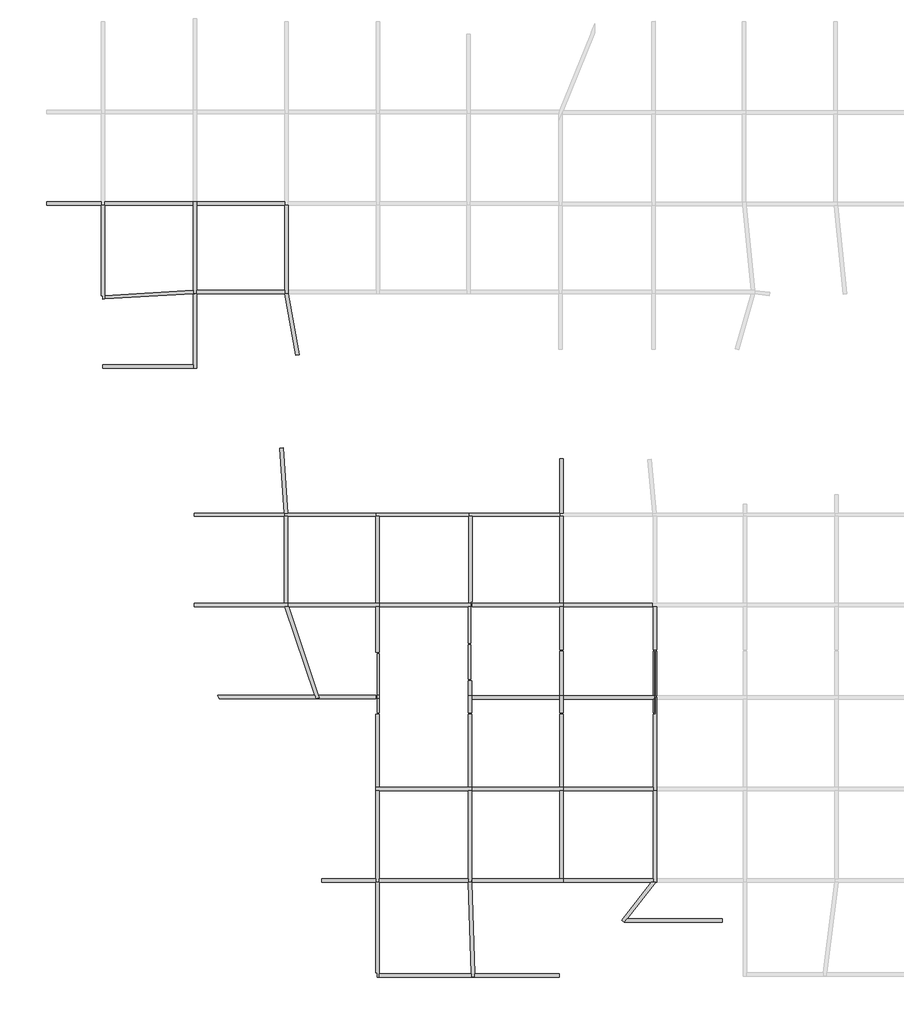
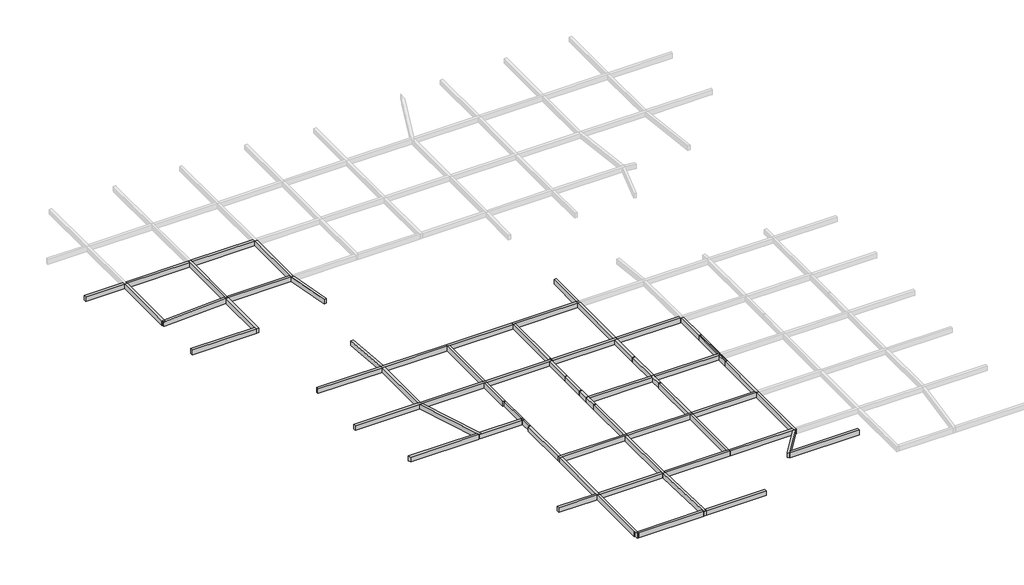
# One storey, part 1 of 8: 56 beams.
"""IFC4 building model written with IfcOpenShell, lengths in millimetres."""

import ifcopenshell
import ifcopenshell.guid

model = None  # the IFC model being written
_history = None  # IfcOwnerHistory: only IFC2X3 demands one
_inside = {}  # id of a spatial element -> (the spatial element, [elements in it])
_under = {}  # id of a project, library or spatial element -> (it, [spatial elements below it])
_declared = {}  # id of a project -> (the project, [libraries it declares])
_typed = {}  # id of a type object -> (the type object, [elements of that type])
_made_of = {}  # id of a material, layer set ... -> (it, [elements and type objects made of it])


def new_model(schema):
    """Start an empty IFC model of exactly this schema.

    Asked for "IFC4X3", IfcOpenShell would pick the latest addendum, in which some entities
    have other attributes; the version numbers below select the first issue.
    IFC2X3 requires an IfcOwnerHistory on every rooted entity: one is made here for all.
    """
    global model, _history
    if schema == "IFC4X3":
        model = ifcopenshell.file(schema_version=(4, 3, 0, 0))
    else:
        model = ifcopenshell.file(schema=schema)
    _inside.clear()
    _under.clear()
    _declared.clear()
    _typed.clear()
    _made_of.clear()
    _history = None
    if model.schema == "IFC2X3":
        org = make("IfcOrganization", Name="unknown")
        user = make(
            "IfcPersonAndOrganization",
            ThePerson=make("IfcPerson", FamilyName="unknown"),
            TheOrganization=org,
        )
        app = make(
            "IfcApplication",
            ApplicationDeveloper=org,
            Version="unknown",
            ApplicationFullName="unknown",
            ApplicationIdentifier="unknown",
        )
        _history = make(
            "IfcOwnerHistory",
            OwningUser=user,
            OwningApplication=app,
            ChangeAction="ADDED",
            CreationDate=0,
        )
    return model


def make(cls, **values):
    """One entity of the class cls with the attributes given. An attribute that is None is left unset."""
    return model.create_entity(
        cls, **{name: value for name, value in values.items() if value is not None}
    )


def rooted(cls, **values):
    """An entity with a GlobalId (a new one), such as an element, a storey or a relation."""
    return make(cls, GlobalId=ifcopenshell.guid.new(), OwnerHistory=_history, **values)


def si_unit(unit_type, name, prefix=None):
    """IfcSIUnit, for example si_unit("LENGTHUNIT", "METRE", prefix="MILLI")."""
    return make("IfcSIUnit", UnitType=unit_type, Prefix=prefix, Name=name)


def assignment(units):
    """IfcUnitAssignment: the units of a project."""
    return None if units is None else make("IfcUnitAssignment", Units=units)


def point(xyz):
    """IfcCartesianPoint."""
    return None if xyz is None else make("IfcCartesianPoint", Coordinates=xyz)


def direction(xyz):
    """IfcDirection."""
    return None if xyz is None else make("IfcDirection", DirectionRatios=xyz)


def frame(location, z_axis=None, x_axis=None):
    """IfcAxis2Placement3D, a coordinate frame: its origin and axes. An axis left out is left unset."""
    return make(
        "IfcAxis2Placement3D",
        Location=point(location),
        Axis=direction(z_axis),
        RefDirection=direction(x_axis),
    )


def origin():
    """The frame at (0, 0, 0) with its axes left unset."""
    return frame((0.0, 0.0, 0.0))


def place(relative_to, where):
    """IfcLocalPlacement: puts the frame where relative to a parent placement (None: the world)."""
    return make(
        "IfcLocalPlacement", PlacementRelTo=relative_to, RelativePlacement=where
    )


def context(
    kind, dimensions, precision=None, world=None, true_north=None, identifier=None
):
    """IfcGeometricRepresentationContext, for example the 3D "Model" context."""
    return make(
        "IfcGeometricRepresentationContext",
        ContextIdentifier=identifier,
        ContextType=kind,
        CoordinateSpaceDimension=dimensions,
        Precision=precision,
        WorldCoordinateSystem=world,
        TrueNorth=true_north,
    )


def project(units=None, contexts=None):
    """IfcProject with its units and contexts."""
    return rooted(
        "IfcProject",
        Name="project",
        RepresentationContexts=contexts,
        UnitsInContext=assignment(units),
    )


def spatial(cls, under=None, at=None, **own):
    """A site, building, storey or space (cls), placed at a placement, below another one or the project."""
    s = rooted(cls, ObjectPlacement=at, **own)
    if under is not None:
        _under.setdefault(under.id(), (under, []))[1].append(s)
    return s


def polyline(points):
    """IfcPolyline through the points."""
    return make("IfcPolyline", Points=[point(p) for p in points])


def outline(outer, holes=None, kind="AREA"):
    """IfcArbitraryClosedProfileDef: a profile drawn as a closed curve; with holes, ...WithVoids."""
    if holes is None:
        return make("IfcArbitraryClosedProfileDef", ProfileType=kind, OuterCurve=outer)
    return make(
        "IfcArbitraryProfileDefWithVoids",
        ProfileType=kind,
        OuterCurve=outer,
        InnerCurves=holes,
    )


def extrude(swept, where, along, depth):
    """IfcExtrudedAreaSolid: the profile swept, set in the frame where, extruded along a direction by depth."""
    return make(
        "IfcExtrudedAreaSolid",
        SweptArea=swept,
        Position=where,
        ExtrudedDirection=direction(along),
        Depth=depth,
    )


def faces_of(points, faces, orient=None, outer=None):
    """IfcFace entities. A face is a list of loops; a loop is a list of indices into points, from 0.

    orient and outer hold one flag for each loop. By default every Orientation is true, the
    first loop of a face is its IfcFaceOuterBound and the others are IfcFaceBound.
    """
    made = []
    for i, loops in enumerate(faces):
        bounds = []
        for j, loop in enumerate(loops):
            is_outer = j == 0 if outer is None else outer[i][j]
            bounds.append(
                make(
                    "IfcFaceOuterBound" if is_outer else "IfcFaceBound",
                    Bound=make("IfcPolyLoop", Polygon=[points[k] for k in loop]),
                    Orientation=True if orient is None else orient[i][j],
                )
            )
        made.append(make("IfcFace", Bounds=bounds))
    return made


def faceted_brep(points, faces, orient=None, outer=None, voids=None):
    """IfcFacetedBrep: a solid bounded by flat faces; with voids (closed shells), ...WithVoids."""
    shared = [point(p) for p in points]
    hull = make("IfcClosedShell", CfsFaces=faces_of(shared, faces, orient, outer))
    if voids is None:
        return make("IfcFacetedBrep", Outer=hull)
    return make(
        "IfcFacetedBrepWithVoids",
        Outer=hull,
        Voids=[
            make(cls, CfsFaces=faces_of(shared, fs, o, b)) for cls, fs, o, b in voids
        ],
    )


def shape(context_of_items, identifier, shape_type, items):
    """IfcShapeRepresentation: the items that make up one representation, for example the "Body"."""
    return make(
        "IfcShapeRepresentation",
        ContextOfItems=context_of_items,
        RepresentationIdentifier=identifier,
        RepresentationType=shape_type,
        Items=items,
    )


def made_of(thing, what):
    """Note that an element or type object is made of a material, layer set ...; save() writes the relation."""
    if what is not None:
        _made_of.setdefault(what.id(), (what, []))[1].append(thing)
    return thing


def element(
    cls,
    number,
    at=None,
    inside=None,
    cuts=None,
    type_object=None,
    material=None,
    context=None,
    identifier="Body",
    shape_type=None,
    held_by="IfcProductDefinitionShape",
    body=None,
    shapes=None,
    **own,
):
    """One element of the class cls, such as IfcWall. Its Tag is "e" and its number.

    at: its placement. inside: the storey or other place that contains it. cuts: it is an
    opening in that element (IfcRelVoidsElement). A single representation is given by context,
    identifier, shape_type and body (its items); several are given by shapes. held_by: the class
    of the entity that holds the representations. save() writes the other relations.
    """
    e = rooted(cls, Tag="e%d" % number, ObjectPlacement=at, **own)
    if body is not None:
        shapes = [shape(context, identifier, shape_type, body)]
    if shapes is not None:
        e.Representation = make(held_by, Representations=shapes)
    if inside is not None:
        _inside.setdefault(inside.id(), (inside, []))[1].append(e)
    if cuts is not None:
        rooted(
            "IfcRelVoidsElement", RelatingBuildingElement=cuts, RelatedOpeningElement=e
        )
    if type_object is not None:
        _typed.setdefault(type_object.id(), (type_object, []))[1].append(e)
    return made_of(e, material)


def aggregate(whole, parts):
    """IfcRelAggregates: a whole, such as a stair, and the parts it consists of."""
    return rooted("IfcRelAggregates", RelatingObject=whole, RelatedObjects=parts)


def save(model, path):
    """Write the relations noted so far, then the file.

    IfcRelAggregates (storeys below a building ...), IfcRelContainedInSpatialStructure (elements
    in a storey), IfcRelDefinesByType, IfcRelAssociatesMaterial and IfcRelDeclares: one each for
    every whole, place, type object, material and project.
    """
    for whole, parts in _under.values():
        aggregate(whole, parts)
    for where, things in _inside.values():
        rooted(
            "IfcRelContainedInSpatialStructure",
            RelatedElements=things,
            RelatingStructure=where,
        )
    for kind, things in _typed.values():
        rooted("IfcRelDefinesByType", RelatedObjects=things, RelatingType=kind)
    for what, things in _made_of.values():
        rooted("IfcRelAssociatesMaterial", RelatedObjects=things, RelatingMaterial=what)
    for by, libraries in _declared.values():
        rooted("IfcRelDeclares", RelatingContext=by, RelatedDefinitions=libraries)
    model.write(path)


model = new_model("IFC4")

# Units and contexts
model_context = context("Model", 3, world=origin())
ifc_project = project(units=[si_unit("LENGTHUNIT", "METRE", prefix="MILLI")], contexts=[model_context])

# Site, building, storey
site = spatial("IfcSite", under=ifc_project)
building = spatial("IfcBuilding", under=site)
storey = spatial("IfcBuildingStorey", under=building, Name="层高", Elevation=3300.0)

# Beams
placement = place(None, origin())
element("IfcBeam", 1, ObjectType="混凝土 - 矩形梁 : KL_beam", at=placement, inside=storey, context=model_context, shape_type="SweptSolid", body=[
    extrude(outline(polyline([(73233.8430954, 95377.0451941), (73233.8430954, 95677.0451941), (77970.8225114, 95677.0451941), (77970.8225114, 95377.0451941), (73233.8430954, 95377.0451941)])), frame((0.0, 0.0, 2700.0), z_axis=(0.0, 0.0, 1.0), x_axis=(1.0, 0.0, 0.0)), (0.0, 0.0, 1.0), 600.0),
])
element("IfcBeam", 2, ObjectType="混凝土 - 矩形梁 : KL_beam", at=placement, inside=storey, context=model_context, shape_type="Brep", body=[
    faceted_brep([(78270.8225114, 95377.0451941, 3300.0), (77970.8225114, 95377.0451941, 3300.0), (77970.8225114, 87547.0451941, 3300.0), (78083.8475536, 87547.0451941, 3300.0), (78083.8475536, 87427.0451941, 3300.0), (78083.8475536, 87285.4298587, 3300.0), (78270.8225114, 87285.4298587, 3300.0), (78270.8225114, 87585.9262923, 3300.0), (77970.8225114, 95377.0451941, 2700.0), (78270.8225114, 95377.0451941, 2700.0), (78270.8225114, 87585.9262923, 2700.0), (78270.8225114, 87285.4298587, 2700.0), (78083.8475536, 87285.4298587, 2700.0), (78083.8475536, 87547.0451941, 2700.0), (77970.8225114, 87547.0451941, 2700.0)], [[[0, 1, 2, 3, 4, 5, 6, 7]], [[8, 9, 10, 11, 12, 13, 14]], [[9, 0, 7, 6, 11, 10]], [[1, 0, 9, 8]], [[13, 3, 2, 14]], [[3, 13, 12, 5, 4]], [[11, 6, 5, 12]], [[1, 8, 14, 2]]]),
])
element("IfcBeam", 3, ObjectType="混凝土 - 矩形梁 : KL_beam", at=placement, inside=storey, context=model_context, shape_type="Brep", body=[
    faceted_brep([(86170.8225114, 95677.0451941, 3300.0), (85870.8225114, 95677.0451941, 3300.0), (85870.8225114, 95377.0451941, 3300.0), (85870.8225114, 88023.3256155, 3300.0), (85870.8225114, 87731.7102801, 3300.0), (86025.1353836, 87731.7102801, 3300.0), (86170.8225114, 87731.7102801, 3300.0), (86170.8225114, 88031.7102801, 3300.0), (86170.8225114, 95377.0451941, 3300.0), (86170.8225114, 95677.0451941, 2700.0), (86170.8225114, 87731.7102801, 2700.0), (86170.8225114, 88031.7102801, 2700.0), (86170.8225114, 95377.0451941, 2700.0), (85870.8225114, 95677.0451941, 2700.0), (86025.1353836, 87731.7102801, 2700.0), (85870.8225114, 87731.7102801, 2700.0), (85870.8225114, 88023.3256155, 2700.0), (85870.8225114, 95377.0451941, 2700.0)], [[[0, 1, 2, 3, 4, 5, 6, 7, 8]], [[9, 0, 8, 7, 6, 10, 11, 12]], [[13, 9, 12, 11, 10, 14, 15, 16, 17]], [[1, 13, 17, 16, 15, 4, 3, 2]], [[1, 0, 9, 13]], [[6, 5, 4, 15, 14, 10]]]),
])
element("IfcBeam", 4, ObjectType="混凝土 - 矩形梁 : KL_beam", at=placement, inside=storey, context=model_context, shape_type="Brep", body=[
    faceted_brep([(93770.8225114, 87731.7102801, 3300.0), (93794.9575667, 87731.7102801, 3300.0), (94070.8225114, 87731.7102801, 3300.0), (94070.8225114, 88031.7102801, 3300.0), (94070.8225114, 95377.0451941, 3300.0), (93770.8225114, 95377.0451941, 3300.0), (93770.8225114, 88031.7102801, 3300.0), (93770.8225114, 87731.7102801, 2700.0), (93770.8225114, 95377.0451941, 2700.0), (93770.8225114, 88031.7102801, 2700.0), (94070.8225114, 87731.7102801, 2700.0), (93794.9575667, 87731.7102801, 2700.0), (94070.8225114, 95377.0451941, 2700.0), (94070.8225114, 88031.7102801, 2700.0)], [[[0, 1, 2, 3, 4, 5, 6]], [[7, 0, 6, 5, 8, 9]], [[10, 11, 7, 9, 8, 12, 13]], [[2, 10, 13, 12, 4, 3]], [[5, 4, 12, 8]], [[2, 1, 0, 7, 11, 10]]]),
])
element("IfcBeam", 5, ObjectType="混凝土 - 矩形梁 : KL_beam", at=placement, inside=storey, context=model_context, shape_type="Brep", body=[
    faceted_brep([(109648.7128309, 68825.8567488, 3300.0), (109648.7128309, 68525.8567488, 3300.0), (109948.7128309, 68525.8567488, 3300.0), (117498.8477351, 68525.8567488, 3300.0), (117498.8477351, 68825.8567488, 3300.0), (109648.7128309, 68825.8567488, 2700.0), (117498.8477351, 68825.8567488, 2700.0), (109648.7128309, 68525.8567488, 2700.0), (117498.8477351, 68525.8567488, 2700.0), (109948.7128309, 68525.8567488, 2700.0)], [[[0, 1, 2, 3, 4]], [[5, 0, 4, 6]], [[7, 5, 6, 8, 9]], [[1, 7, 9, 8, 3, 2]], [[1, 0, 5, 7]], [[4, 3, 8, 6]]]),
])
element("IfcBeam", 6, ObjectType="混凝土 - 矩形梁 : KL_beam", at=placement, inside=storey, context=model_context, shape_type="Brep", body=[
    faceted_brep([(101648.7128309, 68825.8567488, 3300.0), (101648.7128309, 68525.8567488, 3300.0), (101948.7128309, 68525.8567488, 3300.0), (109648.7128309, 68525.8567488, 3300.0), (109648.7128309, 68825.8567488, 3300.0), (101648.7128309, 68825.8567488, 2700.0), (109648.7128309, 68825.8567488, 2700.0), (101648.7128309, 68525.8567488, 2700.0), (109648.7128309, 68525.8567488, 2700.0), (101948.7128309, 68525.8567488, 2700.0)], [[[0, 1, 2, 3, 4]], [[5, 0, 4, 6]], [[7, 5, 6, 8, 9]], [[1, 7, 9, 8, 3, 2]], [[4, 3, 8, 6]], [[1, 0, 5, 7]]]),
])
element("IfcBeam", 7, ObjectType="混凝土 - 矩形梁 : KL_beam", at=placement, inside=storey, context=model_context, shape_type="Brep", body=[
    faceted_brep([(93748.7128309, 68825.8567488, 3300.0), (93748.7128309, 68525.8567488, 3300.0), (94048.7128309, 68525.8567488, 3300.0), (101648.7128309, 68525.8567488, 3300.0), (101648.7128309, 68825.8567488, 3300.0), (94038.5900938, 68825.8567488, 3300.0), (93748.7128309, 68825.8567488, 2700.0), (101648.7128309, 68825.8567488, 2700.0), (94038.5900938, 68825.8567488, 2700.0), (93748.7128309, 68525.8567488, 2700.0), (101648.7128309, 68525.8567488, 2700.0), (94048.7128309, 68525.8567488, 2700.0)], [[[0, 1, 2, 3, 4, 5]], [[6, 0, 5, 4, 7, 8]], [[9, 6, 8, 7, 10, 11]], [[1, 9, 11, 10, 3, 2]], [[4, 3, 10, 7]], [[1, 0, 6, 9]]]),
])
element("IfcBeam", 8, ObjectType="混凝土 - 矩形梁 : KL_beam", at=placement, inside=storey, context=model_context, shape_type="Brep", body=[
    faceted_brep([(85958.8477345, 68825.8567488, 3300.0), (85958.8477345, 68525.8567488, 3300.0), (93748.7128309, 68525.8567488, 3300.0), (93748.7128309, 68825.8567488, 3300.0), (93737.8575244, 68825.8567488, 3300.0), (85958.8477345, 68825.8567488, 2700.0), (93748.7128309, 68825.8567488, 2700.0), (93737.8575244, 68825.8567488, 2700.0), (85958.8477345, 68525.8567488, 2700.0), (93748.7128309, 68525.8567488, 2700.0)], [[[0, 1, 2, 3, 4]], [[5, 0, 4, 3, 6, 7]], [[8, 5, 7, 6, 9]], [[1, 8, 9, 2]], [[1, 0, 5, 8]], [[3, 2, 9, 6]]]),
])
element("IfcBeam", 9, ObjectType="混凝土 - 矩形梁 : KL_beam", at=placement, inside=storey, context=model_context, shape_type="Brep", body=[
    faceted_brep([(94048.7128309, 60727.1438632, 3300.0), (94048.7128309, 61027.1438632, 3300.0), (93748.7128309, 61027.1438632, 3300.0), (85958.8477345, 61027.1438632, 3300.0), (85958.8477345, 60727.1438632, 3300.0), (93791.0953712, 60727.1438632, 3300.0), (94048.7128309, 60727.1438632, 2700.0), (85958.8477345, 60727.1438632, 2700.0), (93791.0953712, 60727.1438632, 2700.0), (94048.7128309, 61027.1438632, 2700.0), (85958.8477345, 61027.1438632, 2700.0), (93748.7128309, 61027.1438632, 2700.0)], [[[0, 1, 2, 3, 4, 5]], [[6, 0, 5, 4, 7, 8]], [[9, 6, 8, 7, 10, 11]], [[1, 9, 11, 10, 3, 2]], [[4, 3, 10, 7]], [[1, 0, 6, 9]]]),
])
element("IfcBeam", 10, ObjectType="混凝土 - 矩形梁 : KL_beam", at=placement, inside=storey, context=model_context, shape_type="Brep", body=[
    faceted_brep([(101948.7128309, 60727.1438632, 3300.0), (101948.7128309, 61027.1438632, 3300.0), (101648.7128309, 61027.1438632, 3300.0), (94048.7128309, 61027.1438632, 3300.0), (94048.7128309, 60727.1438632, 3300.0), (94107.7867122, 60727.1438632, 3300.0), (101648.7128309, 60727.1438632, 3300.0), (101948.7128309, 60727.1438632, 2700.0), (94048.7128309, 60727.1438632, 2700.0), (94107.7867122, 60727.1438632, 2700.0), (101648.7128309, 60727.1438632, 2700.0), (101948.7128309, 61027.1438632, 2700.0), (94048.7128309, 61027.1438632, 2700.0), (101648.7128309, 61027.1438632, 2700.0)], [[[0, 1, 2, 3, 4, 5, 6]], [[7, 0, 6, 5, 4, 8, 9, 10]], [[11, 7, 10, 9, 8, 12, 13]], [[1, 11, 13, 12, 3, 2]], [[1, 0, 7, 11]], [[4, 3, 12, 8]]]),
])
element("IfcBeam", 11, ObjectType="混凝土 - 矩形梁 : KL_beam", at=placement, inside=storey, context=model_context, shape_type="Brep", body=[
    faceted_brep([(101948.7128309, 61027.1438632, 3300.0), (101948.7128309, 60727.1438632, 3300.0), (109598.8477351, 60727.1438632, 3300.0), (109838.7128377, 60727.1438632, 3300.0), (109838.7128377, 61027.1438632, 3300.0), (109648.7128309, 61027.1438632, 3300.0), (101948.7128309, 60727.1438632, 2700.0), (109598.8477351, 60727.1438632, 2700.0), (109838.7128377, 60727.1438632, 2700.0), (101948.7128309, 61027.1438632, 2700.0), (109648.7128309, 61027.1438632, 2700.0), (109838.7128377, 61027.1438632, 2700.0)], [[[0, 1, 2, 3, 4, 5]], [[1, 6, 7, 8, 3, 2]], [[6, 9, 10, 11, 8, 7]], [[9, 0, 5, 4, 11, 10]], [[1, 0, 9, 6]], [[4, 3, 8, 11]]]),
])
element("IfcBeam", 12, ObjectType="混凝土 - 矩形梁 : KL_beam", at=placement, inside=storey, context=model_context, shape_type="Brep", body=[
    faceted_brep([(117798.8477351, 60727.1438632, 3300.0), (117798.8477351, 61027.1438632, 3300.0), (117498.8477351, 61027.1438632, 3300.0), (109958.7128377, 61027.1438632, 3300.0), (109958.7128377, 60727.1438632, 3300.0), (117498.8477351, 60727.1438632, 3300.0), (117798.8477351, 60727.1438632, 2700.0), (109958.7128377, 60727.1438632, 2700.0), (117498.8477351, 60727.1438632, 2700.0), (117798.8477351, 61027.1438632, 2700.0), (109958.7128377, 61027.1438632, 2700.0), (117498.8477351, 61027.1438632, 2700.0)], [[[0, 1, 2, 3, 4, 5]], [[6, 0, 5, 4, 7, 8]], [[9, 6, 8, 7, 10, 11]], [[1, 9, 11, 10, 3, 2]], [[1, 0, 6, 9]], [[4, 3, 10, 7]]]),
])
element("IfcBeam", 13, ObjectType="混凝土 - 矩形梁 : KL_beam", at=placement, inside=storey, context=model_context, shape_type="SweptSolid", body=[
    extrude(outline(polyline([(125476.4248507, 61027.1438632), (125476.4248507, 60727.1438632), (117798.8477351, 60727.1438632), (117798.8477351, 61027.1438632), (125476.4248507, 61027.1438632)])), frame((0.0, 0.0, 2700.0), z_axis=(0.0, 0.0, 1.0), x_axis=(1.0, 0.0, 0.0)), (0.0, 0.0, 1.0), 600.0),
])
element("IfcBeam", 14, ObjectType="混凝土 - 矩形梁 : KL_beam", at=placement, inside=storey, context=model_context, shape_type="SweptSolid", body=[
    extrude(outline(polyline([(109648.7128309, 68525.8567488), (109948.7128309, 68525.8567488), (109948.7128309, 61154.2483952), (109838.7128377, 61154.2483952), (109838.7128377, 61027.1438632), (109648.7128309, 61027.1438632), (109648.7128309, 68525.8567488)])), frame((0.0, 0.0, 2700.0), z_axis=(0.0, 0.0, 1.0), x_axis=(1.0, 0.0, 0.0)), (0.0, 0.0, 1.0), 600.0),
])
element("IfcBeam", 15, ObjectType="混凝土 - 矩形梁 : KL_beam", at=placement, inside=storey, context=model_context, shape_type="SweptSolid", body=[
    extrude(outline(polyline([(101648.7128309, 68525.8567488), (101948.7128309, 68525.8567488), (101948.7128309, 61027.1438632), (101648.7128309, 61027.1438632), (101648.7128309, 68525.8567488)])), frame((0.0, 0.0, 2700.0), z_axis=(0.0, 0.0, 1.0), x_axis=(1.0, 0.0, 0.0)), (0.0, 0.0, 1.0), 600.0),
])
element("IfcBeam", 16, ObjectType="混凝土 - 矩形梁 : KL_beam", at=placement, inside=storey, context=model_context, shape_type="SweptSolid", body=[
    extrude(outline(polyline([(93748.7128309, 68525.8567488), (94048.7128309, 68525.8567488), (94048.7128309, 61027.1438632), (93748.7128309, 61027.1438632), (93748.7128309, 68525.8567488)])), frame((0.0, 0.0, 2700.0), z_axis=(0.0, 0.0, 1.0), x_axis=(1.0, 0.0, 0.0)), (0.0, 0.0, 1.0), 600.0),
])
element("IfcBeam", 17, ObjectType="混凝土 - 矩形梁 : KL_beam", at=placement, inside=storey, context=model_context, shape_type="Brep", body=[
    faceted_brep([(93345.7815071, 74432.8050195, 3300.0), (93645.0507222, 74453.7319616, 3300.0), (93645.0507222, 74453.7319616, 2700.0), (93345.7815071, 74432.8050195, 2700.0), (93737.8575244, 68825.8567488, 3300.0), (93748.7128309, 68825.8567488, 3300.0), (94038.5900938, 68825.8567488, 3300.0), (94038.5900938, 68825.8567488, 2700.0), (93748.7128309, 68825.8567488, 2700.0), (93737.8575244, 68825.8567488, 2700.0)], [[[0, 1, 2, 3]], [[1, 0, 4, 5, 6]], [[2, 1, 6, 7]], [[3, 2, 7, 8, 9]], [[0, 3, 9, 4]], [[4, 9, 8, 7, 6, 5]]]),
])
element("IfcBeam", 18, ObjectType="混凝土 - 矩形梁 : KL_beam", at=placement, inside=storey, context=model_context, shape_type="Brep", body=[
    faceted_brep([(94107.7867122, 60727.1438632, 3300.0), (94048.7128309, 60727.1438632, 3300.0), (93791.0953712, 60727.1438632, 3300.0), (96364.7738589, 53116.9449825, 3300.0), (96466.2302805, 52816.9449825, 3300.0), (96750.4186632, 52913.0541037, 3300.0), (96681.4652, 53116.9449825, 3300.0), (93791.0953712, 60727.1438632, 2700.0), (96364.7738589, 53116.9449825, 2700.0), (96466.2302805, 52816.9449825, 2700.0), (94048.7128309, 60727.1438632, 2700.0), (94107.7867122, 60727.1438632, 2700.0), (96681.4652, 53116.9449825, 2700.0), (96750.4186632, 52913.0541037, 2700.0)], [[[0, 1, 2, 3, 4, 5, 6]], [[4, 3, 2, 7, 8, 9]], [[9, 8, 7, 10, 11, 12, 13]], [[5, 13, 12, 11, 0, 6]], [[0, 11, 10, 7, 2, 1]], [[5, 4, 9, 13]]]),
])
element("IfcBeam", 19, ObjectType="混凝土 - 矩形梁 : KL_beam", at=placement, inside=storey, context=model_context, shape_type="Brep", body=[
    faceted_brep([(88137.9209142, 52816.9449825, 3300.0), (96423.8477403, 52816.9449825, 3300.0), (96466.2302805, 52816.9449825, 3300.0), (96364.7738589, 53116.9449825, 3300.0), (88016.7130465, 53116.9449825, 3300.0), (88016.7130465, 53116.9449825, 2700.0), (96364.7738589, 53116.9449825, 2700.0), (96466.2302805, 52816.9449825, 2700.0), (96423.8477403, 52816.9449825, 2700.0), (88137.9209142, 52816.9449825, 2700.0)], [[[0, 1, 2, 3, 4]], [[5, 4, 3, 6]], [[7, 8, 9, 5, 6]], [[2, 1, 0, 9, 8, 7]], [[0, 4, 5, 9]], [[3, 2, 7, 6]]]),
])
element("IfcBeam", 20, ObjectType="混凝土 - 矩形梁 : KL_beam", at=placement, inside=storey, context=model_context, shape_type="Brep", body=[
    faceted_brep([(101948.7128309, 52816.9449825, 3300.0), (101948.7128309, 53116.9449825, 3300.0), (101758.8477337, 53116.9449825, 3300.0), (101758.8477337, 52816.9449825, 3300.0), (101948.7128309, 52816.9449825, 2700.0), (101758.8477337, 52816.9449825, 2700.0), (101948.7128309, 53116.9449825, 2700.0), (101758.8477337, 53116.9449825, 2700.0)], [[[0, 1, 2, 3]], [[4, 0, 3, 5]], [[6, 4, 5, 7]], [[1, 6, 7, 2]], [[1, 0, 4, 6]], [[3, 2, 7, 5]]]),
    faceted_brep([(96750.4186632, 52913.0541037, 2700.0), (96750.4186632, 52913.0541037, 3300.0), (96681.4652, 53116.9449825, 3300.0), (96681.4652, 53116.9449825, 2700.0), (96466.2302805, 52816.9449825, 2700.0), (96466.2302805, 52816.9449825, 3300.0), (101638.8477337, 53116.9449825, 3300.0), (101638.8477337, 52816.9449825, 3300.0), (101638.8477337, 52816.9449825, 2700.0), (101638.8477337, 53116.9449825, 2700.0), (96723.8477403, 52816.9449825, 3300.0), (96723.8477403, 52816.9449825, 2700.0)], [[[0, 1, 2, 3]], [[1, 0, 4, 5]], [[6, 7, 8, 9]], [[2, 1, 5, 10, 7, 6]], [[5, 4, 11, 8, 7, 10]], [[0, 3, 9, 8, 11, 4]], [[3, 2, 6, 9]]]),
])
element("IfcBeam", 21, ObjectType="混凝土 - 矩形梁 : KL_beam", at=placement, inside=storey, context=model_context, shape_type="Brep", body=[
    faceted_brep([(109898.8477351, 44882.6668088, 3300.0), (109898.8477351, 45182.6668088, 3300.0), (109598.8477351, 45182.6668088, 3300.0), (101948.7128309, 45182.6668088, 3300.0), (101648.7128309, 45182.6668088, 3300.0), (101648.7128309, 44882.6668088, 3300.0), (101948.7128309, 44882.6668088, 3300.0), (109598.8477351, 44882.6668088, 3300.0), (109898.8477351, 44882.6668088, 2700.0), (101648.7128309, 44882.6668088, 2700.0), (101948.7128309, 44882.6668088, 2700.0), (109598.8477351, 44882.6668088, 2700.0), (109898.8477351, 45182.6668088, 2700.0), (101648.7128309, 45182.6668088, 2700.0), (101948.7128309, 45182.6668088, 2700.0), (109598.8477351, 45182.6668088, 2700.0)], [[[0, 1, 2, 3, 4, 5, 6, 7]], [[8, 0, 7, 6, 5, 9, 10, 11]], [[12, 8, 11, 10, 9, 13, 14, 15]], [[1, 12, 15, 14, 13, 4, 3, 2]], [[1, 0, 8, 12]], [[5, 4, 13, 9]]]),
])
element("IfcBeam", 22, ObjectType="混凝土 - 矩形梁 : KL_beam", at=placement, inside=storey, context=model_context, shape_type="Brep", body=[
    faceted_brep([(109898.8477351, 53082.6668088, 3300.0), (109598.8477351, 53082.6668088, 3300.0), (109598.8477351, 52816.9449825, 3300.0), (109598.8477351, 51576.8472247, 3300.0), (109898.8477351, 51576.8472247, 3300.0), (109898.8477351, 52782.6668088, 3300.0), (109898.8477351, 53082.6668088, 2700.0), (109898.8477351, 51576.8472247, 2700.0), (109898.8477351, 52782.6668088, 2700.0), (109598.8477351, 53082.6668088, 2700.0), (109598.8477351, 51576.8472247, 2700.0), (109598.8477351, 52816.9449825, 2700.0)], [[[0, 1, 2, 3, 4, 5]], [[6, 0, 5, 4, 7, 8]], [[9, 6, 8, 7, 10, 11]], [[1, 9, 11, 10, 3, 2]], [[1, 0, 6, 9]], [[4, 3, 10, 7]]]),
    faceted_brep([(109898.8477351, 45182.6668088, 3300.0), (109598.8477351, 45182.6668088, 3300.0), (109598.8477351, 45182.6668088, 2700.0), (109898.8477351, 45182.6668088, 2700.0), (109598.8477351, 51456.8472247, 3300.0), (109898.8477351, 51456.8472247, 3300.0), (109898.8477351, 51456.8472247, 2700.0), (109598.8477351, 51456.8472247, 2700.0)], [[[0, 1, 2, 3]], [[4, 5, 6, 7]], [[1, 0, 5, 4]], [[0, 3, 6, 5]], [[3, 2, 7, 6]], [[2, 1, 4, 7]]]),
])
element("IfcBeam", 23, ObjectType="混凝土 - 矩形梁 : KL_beam", at=placement, inside=storey, context=model_context, shape_type="Brep", body=[
    faceted_brep([(109598.8477351, 60727.1438632, 3300.0), (109598.8477351, 57577.1438632, 3300.0), (109838.7128377, 57577.1438632, 3300.0), (109838.7128377, 60727.1438632, 3300.0), (109598.8477351, 57577.1438632, 2700.0), (109598.8477351, 60727.1438632, 2700.0), (109838.7128377, 60727.1438632, 2700.0), (109838.7128377, 57577.1438632, 2700.0)], [[[0, 1, 2, 3]], [[4, 5, 6, 7]], [[0, 5, 4, 1]], [[5, 0, 3, 6]], [[2, 1, 4, 7]], [[3, 2, 7, 6]]]),
    faceted_brep([(109898.8477351, 53082.6668088, 3300.0), (109898.8477351, 53082.6668088, 2700.0), (109898.8477351, 54367.0649839, 2700.0), (109898.8477351, 54367.0649839, 3300.0), (109598.8477351, 53082.6668088, 3300.0), (109598.8477351, 53082.6668088, 2700.0), (109598.8477351, 54367.0649839, 2700.0), (109598.8477351, 54367.0649839, 3300.0), (109598.8477351, 53116.9449825, 3300.0), (109598.8477351, 53116.9449825, 2700.0)], [[[0, 1, 2, 3]], [[0, 4, 5, 1]], [[3, 2, 6, 7]], [[5, 4, 8, 7, 6, 9]], [[4, 0, 3, 7, 8]], [[1, 5, 9, 6, 2]]]),
    faceted_brep([(109598.8477351, 57457.1438632, 3300.0), (109838.7128377, 57457.1438632, 3300.0), (109838.7128377, 57457.1438632, 2700.0), (109598.8477351, 57457.1438632, 2700.0), (109598.8477351, 54487.0649839, 2700.0), (109598.8477351, 54487.0649839, 3300.0), (109838.7128377, 54487.0649839, 3300.0), (109838.7128377, 54487.0649839, 2700.0)], [[[0, 1, 2, 3]], [[0, 3, 4, 5]], [[1, 0, 5, 6]], [[3, 2, 7, 4]], [[1, 6, 7, 2]], [[5, 4, 7, 6]]]),
])
element("IfcBeam", 24, ObjectType="混凝土 - 矩形梁 : KL_beam", at=placement, inside=storey, context=model_context, shape_type="SweptSolid", body=[
    extrude(outline(polyline([(101948.7128309, 56681.8460485), (101948.7128309, 53116.9449825), (101758.8477337, 53116.9449825), (101758.8477337, 56681.8460485), (101948.7128309, 56681.8460485)])), frame((0.0, 0.0, 2700.0), z_axis=(0.0, 0.0, 1.0), x_axis=(1.0, 0.0, 0.0)), (0.0, 0.0, 1.0), 600.0),
    extrude(outline(polyline([(101648.7128309, 60727.1438632), (101948.7128309, 60727.1438632), (101948.7128309, 56801.8460485), (101648.7128309, 56801.8460485), (101648.7128309, 60727.1438632)])), frame((0.0, 0.0, 2700.0), z_axis=(0.0, 0.0, 1.0), x_axis=(1.0, 0.0, 0.0)), (0.0, 0.0, 1.0), 600.0),
])
element("IfcBeam", 25, ObjectType="混凝土 - 矩形梁 : KL_beam", at=placement, inside=storey, context=model_context, shape_type="SweptSolid", body=[
    extrude(outline(polyline([(101948.7128309, 45182.6668088), (101648.7128309, 45182.6668088), (101648.7128309, 51456.8472247), (101948.7128309, 51456.8472247), (101948.7128309, 45182.6668088)])), frame((0.0, 0.0, 2700.0), z_axis=(0.0, 0.0, 1.0), x_axis=(1.0, 0.0, 0.0)), (0.0, 0.0, 1.0), 600.0),
    extrude(outline(polyline([(101948.7128309, 52816.9449825), (101948.7128309, 51576.8472247), (101758.8477337, 51576.8472247), (101758.8477337, 52816.9449825), (101948.7128309, 52816.9449825)])), frame((0.0, 0.0, 2700.0), z_axis=(0.0, 0.0, 1.0), x_axis=(1.0, 0.0, 0.0)), (0.0, 0.0, 1.0), 600.0),
])
element("IfcBeam", 26, ObjectType="混凝土 - 矩形梁 : KL_beam", at=placement, inside=storey, context=model_context, shape_type="Brep", body=[
    faceted_brep([(101648.7128309, 36982.6668088, 3300.0), (101948.7128309, 36982.6668088, 3300.0), (101948.7128309, 37282.6668088, 3300.0), (101948.7128309, 44882.6668088, 3300.0), (101648.7128309, 44882.6668088, 3300.0), (101648.7128309, 37282.6668088, 3300.0), (101648.7128309, 36982.6668088, 2700.0), (101648.7128309, 44882.6668088, 2700.0), (101648.7128309, 37282.6668088, 2700.0), (101948.7128309, 36982.6668088, 2700.0), (101948.7128309, 44882.6668088, 2700.0), (101948.7128309, 37282.6668088, 2700.0)], [[[0, 1, 2, 3, 4, 5]], [[6, 0, 5, 4, 7, 8]], [[9, 6, 8, 7, 10, 11]], [[1, 9, 11, 10, 3, 2]], [[4, 3, 10, 7]], [[1, 0, 6, 9]]]),
])
element("IfcBeam", 27, ObjectType="混凝土 - 矩形梁 : KL_beam", at=placement, inside=storey, context=model_context, shape_type="Brep", body=[
    faceted_brep([(101648.7128309, 29151.649632, 3300.0), (101758.8477432, 29151.649632, 3300.0), (101758.8477432, 29031.649632, 3300.0), (101758.8477432, 28766.8473862, 3300.0), (101948.7128309, 28766.8473862, 3300.0), (101948.7128309, 29066.8473862, 3300.0), (101948.7128309, 36982.6668088, 3300.0), (101648.7128309, 36982.6668088, 3300.0), (101758.8477432, 28766.8473862, 2700.0), (101758.8477432, 29151.649632, 2700.0), (101648.7128309, 29151.649632, 2700.0), (101648.7128309, 36982.6668088, 2700.0), (101948.7128309, 36982.6668088, 2700.0), (101948.7128309, 29066.8473862, 2700.0), (101948.7128309, 28766.8473862, 2700.0)], [[[0, 1, 2, 3, 4, 5, 6, 7]], [[8, 9, 10, 11, 12, 13, 14]], [[12, 6, 5, 4, 14, 13]], [[9, 1, 0, 10]], [[1, 9, 8, 3, 2]], [[10, 0, 7, 11]], [[7, 6, 12, 11]], [[14, 4, 3, 8]]]),
])
element("IfcBeam", 28, ObjectType="混凝土 - 矩形梁 : KL_beam", at=placement, inside=storey, context=model_context, shape_type="SweptSolid", body=[
    extrude(outline(polyline([(96978.261361, 36982.6668088), (96978.261361, 37282.6668088), (101648.7128309, 37282.6668088), (101648.7128309, 36982.6668088), (96978.261361, 36982.6668088)])), frame((0.0, 0.0, 2700.0), z_axis=(0.0, 0.0, 1.0), x_axis=(1.0, 0.0, 0.0)), (0.0, 0.0, 1.0), 600.0),
])
element("IfcBeam", 29, ObjectType="混凝土 - 矩形梁 : KL_beam", at=placement, inside=storey, context=model_context, shape_type="Brep", body=[
    faceted_brep([(109598.8477351, 36982.6668088, 3300.0), (109603.6768872, 36982.6668088, 3300.0), (109898.8477351, 36982.6668088, 3300.0), (109898.8477351, 37135.1208886, 3300.0), (109898.8477351, 37282.6668088, 3300.0), (109898.8477351, 44882.6668088, 3300.0), (109598.8477351, 44882.6668088, 3300.0), (109598.8477351, 37282.6668088, 3300.0), (109598.8477351, 36982.6668088, 2700.0), (109598.8477351, 44882.6668088, 2700.0), (109598.8477351, 37282.6668088, 2700.0), (109898.8477351, 36982.6668088, 2700.0), (109603.6768872, 36982.6668088, 2700.0), (109898.8477351, 44882.6668088, 2700.0), (109898.8477351, 37282.6668088, 2700.0), (109898.8477351, 37135.1208886, 2700.0)], [[[0, 1, 2, 3, 4, 5, 6, 7]], [[8, 0, 7, 6, 9, 10]], [[11, 12, 8, 10, 9, 13, 14, 15]], [[2, 11, 15, 14, 13, 5, 4, 3]], [[6, 5, 13, 9]], [[2, 1, 0, 8, 12, 11]]]),
])
element("IfcBeam", 30, ObjectType="混凝土 - 矩形梁 : KL_beam", at=placement, inside=storey, context=model_context, shape_type="SweptSolid", body=[
    extrude(outline(polyline([(101948.7128309, 36982.6668088), (101948.7128309, 37282.6668088), (109598.8477351, 37282.6668088), (109598.8477351, 36982.6668088), (101948.7128309, 36982.6668088)])), frame((0.0, 0.0, 2700.0), z_axis=(0.0, 0.0, 1.0), x_axis=(1.0, 0.0, 0.0)), (0.0, 0.0, 1.0), 600.0),
])
element("IfcBeam", 31, ObjectType="混凝土 - 矩形梁 : KL_beam", at=placement, inside=storey, context=model_context, shape_type="Brep", body=[
    faceted_brep([(110172.4186602, 28776.6610787, 3300.0), (110162.9209132, 29066.8473862, 3300.0), (109903.8375304, 36982.6668088, 3300.0), (109898.8477351, 37135.1208886, 3300.0), (109898.8477351, 36982.6668088, 3300.0), (109603.6768872, 36982.6668088, 3300.0), (109862.76027, 29066.8473862, 3300.0), (109872.5792174, 28766.8473862, 3300.0), (109603.6768872, 36982.6668088, 2700.0), (109862.76027, 29066.8473862, 2700.0), (109872.5792174, 28766.8473862, 2700.0), (109898.8477351, 36982.6668088, 2700.0), (109898.8477351, 37135.1208886, 2700.0), (109903.8375304, 36982.6668088, 2700.0), (110162.9209132, 29066.8473862, 2700.0), (110172.4186602, 28776.6610787, 2700.0)], [[[0, 1, 2, 3, 4, 5, 6, 7]], [[7, 6, 5, 8, 9, 10]], [[10, 9, 8, 11, 12, 13, 14, 15]], [[3, 2, 1, 0, 15, 14, 13, 12]], [[11, 4, 3, 12]], [[4, 11, 8, 5]], [[0, 7, 10, 15]]]),
])
element("IfcBeam", 32, ObjectType="混凝土 - 矩形梁 : KL_beam", at=placement, inside=storey, context=model_context, shape_type="Brep", body=[
    faceted_brep([(101948.7128309, 29066.8473862, 3300.0), (101948.7128309, 28766.8473862, 3300.0), (109872.5792174, 28766.8473862, 3300.0), (109862.76027, 29066.8473862, 3300.0), (101948.7128309, 29066.8473862, 2700.0), (109862.76027, 29066.8473862, 2700.0), (101948.7128309, 28766.8473862, 2700.0), (109872.5792174, 28766.8473862, 2700.0), (110172.7398606, 28766.8473862, 2700.0), (110172.7398606, 28766.8473862, 3300.0), (110172.4186602, 28776.6610787, 2700.0), (110172.4186602, 28776.6610787, 3300.0)], [[[0, 1, 2, 3]], [[4, 0, 3, 5]], [[6, 4, 5, 7]], [[8, 9, 2, 1, 6, 7]], [[9, 8, 10, 11]], [[1, 0, 4, 6]], [[2, 7, 5, 3]], [[7, 2, 11, 10]], [[9, 11, 2]], [[10, 8, 7]]]),
])
element("IfcBeam", 33, ObjectType="混凝土 - 矩形梁 : KL_beam", at=placement, inside=storey, context=model_context, shape_type="Brep", body=[
    faceted_brep([(117798.8477351, 36982.6668088, 3300.0), (117798.8477351, 37282.6668088, 3300.0), (117498.8477351, 37282.6668088, 3300.0), (109898.8477351, 37282.6668088, 3300.0), (109898.8477351, 37135.1208886, 3300.0), (109903.8375304, 36982.6668088, 3300.0), (117798.8477351, 36982.6668088, 2700.0), (109903.8375304, 36982.6668088, 2700.0), (117798.8477351, 37282.6668088, 2700.0), (109898.8477351, 37135.1208886, 2700.0), (109898.8477351, 37282.6668088, 2700.0), (117498.8477351, 37282.6668088, 2700.0)], [[[0, 1, 2, 3, 4, 5]], [[6, 0, 5, 7]], [[8, 6, 7, 9, 10, 11]], [[10, 3, 2, 1, 8, 11]], [[3, 10, 9, 4]], [[5, 4, 9, 7]], [[1, 0, 6, 8]]]),
])
element("IfcBeam", 34, ObjectType="混凝土 - 矩形梁 : KL_beam", at=placement, inside=storey, context=model_context, shape_type="Brep", body=[
    faceted_brep([(117448.7988991, 29066.8473862, 3300.0), (117448.7988991, 28766.8473862, 3300.0), (117448.7988991, 28766.8473862, 2700.0), (117448.7988991, 29066.8473862, 2700.0), (110162.9209132, 29066.8473862, 3300.0), (110172.4186602, 28776.6610787, 3300.0), (110172.7398606, 28766.8473862, 3300.0), (110172.7398606, 28766.8473862, 2700.0), (110172.4186602, 28776.6610787, 2700.0), (110162.9209132, 29066.8473862, 2700.0)], [[[0, 1, 2, 3]], [[1, 0, 4, 5, 6]], [[2, 1, 6, 7]], [[3, 2, 7, 8, 9]], [[0, 3, 9, 4]], [[4, 9, 8, 7, 6, 5]]]),
])
element("IfcBeam", 35, ObjectType="混凝土 - 矩形梁 : KL_beam", at=placement, inside=storey, context=model_context, shape_type="Brep", body=[
    faceted_brep([(117798.8477351, 44882.6668088, 3300.0), (117798.8477351, 45182.6668088, 3300.0), (117498.8477351, 45182.6668088, 3300.0), (109898.8477351, 45182.6668088, 3300.0), (109898.8477351, 44882.6668088, 3300.0), (117498.8477351, 44882.6668088, 3300.0), (117798.8477351, 44882.6668088, 2700.0), (109898.8477351, 44882.6668088, 2700.0), (117498.8477351, 44882.6668088, 2700.0), (117798.8477351, 45182.6668088, 2700.0), (109898.8477351, 45182.6668088, 2700.0), (117498.8477351, 45182.6668088, 2700.0)], [[[0, 1, 2, 3, 4, 5]], [[6, 0, 5, 4, 7, 8]], [[9, 6, 8, 7, 10, 11]], [[1, 9, 11, 10, 3, 2]], [[4, 3, 10, 7]], [[1, 0, 6, 9]]]),
])
element("IfcBeam", 36, ObjectType="混凝土 - 矩形梁 : KL_beam", at=placement, inside=storey, context=model_context, shape_type="SweptSolid", body=[
    extrude(outline(polyline([(117498.8477351, 44882.6668088), (117798.8477351, 44882.6668088), (117798.8477351, 37282.6668088), (117498.8477351, 37282.6668088), (117498.8477351, 44882.6668088)])), frame((0.0, 0.0, 2700.0), z_axis=(0.0, 0.0, 1.0), x_axis=(1.0, 0.0, 0.0)), (0.0, 0.0, 1.0), 600.0),
])
element("IfcBeam", 37, ObjectType="混凝土 - 矩形梁 : KL_beam", at=placement, inside=storey, context=model_context, shape_type="Brep", body=[
    faceted_brep([(117798.8477351, 53082.6668088, 3300.0), (117498.8477351, 53082.6668088, 3300.0), (117498.8477351, 52782.6668088, 3300.0), (117498.8477351, 51576.8472247, 3300.0), (117798.8477351, 51576.8472247, 3300.0), (117798.8477351, 52782.6668088, 3300.0), (117798.8477351, 53082.6668088, 2700.0), (117798.8477351, 51576.8472247, 2700.0), (117798.8477351, 52782.6668088, 2700.0), (117498.8477351, 53082.6668088, 2700.0), (117498.8477351, 51576.8472247, 2700.0), (117498.8477351, 52782.6668088, 2700.0)], [[[0, 1, 2, 3, 4, 5]], [[6, 0, 5, 4, 7, 8]], [[9, 6, 8, 7, 10, 11]], [[1, 9, 11, 10, 3, 2]], [[1, 0, 6, 9]], [[4, 3, 10, 7]]]),
    faceted_brep([(117798.8477351, 45182.6668088, 3300.0), (117498.8477351, 45182.6668088, 3300.0), (117498.8477351, 45182.6668088, 2700.0), (117798.8477351, 45182.6668088, 2700.0), (117498.8477351, 51456.8472247, 3300.0), (117798.8477351, 51456.8472247, 3300.0), (117798.8477351, 51456.8472247, 2700.0), (117498.8477351, 51456.8472247, 2700.0)], [[[0, 1, 2, 3]], [[4, 5, 6, 7]], [[1, 0, 5, 4]], [[0, 3, 6, 5]], [[3, 2, 7, 6]], [[2, 1, 4, 7]]]),
])
element("IfcBeam", 38, ObjectType="混凝土 - 矩形梁 : KL_beam", at=placement, inside=storey, context=model_context, shape_type="SweptSolid", body=[
    extrude(outline(polyline([(109898.8477351, 52782.6668088), (109898.8477351, 53082.6668088), (117498.8477351, 53082.6668088), (117498.8477351, 52782.6668088), (109898.8477351, 52782.6668088)])), frame((0.0, 0.0, 2700.0), z_axis=(0.0, 0.0, 1.0), x_axis=(1.0, 0.0, 0.0)), (0.0, 0.0, 1.0), 600.0),
])
element("IfcBeam", 39, ObjectType="混凝土 - 矩形梁 : KL_beam", at=placement, inside=storey, context=model_context, shape_type="Brep", body=[
    faceted_brep([(117798.8477351, 53082.6668088, 3300.0), (117798.8477351, 52782.6668088, 3300.0), (125548.8240412, 52782.6668088, 3300.0), (125638.8240412, 52782.6668088, 3300.0), (125638.8240412, 53082.6668088, 3300.0), (125548.8240412, 53082.6668088, 3300.0), (117798.8477351, 52782.6668088, 2700.0), (125548.8240412, 52782.6668088, 2700.0), (125638.8240412, 52782.6668088, 2700.0), (117798.8477351, 53082.6668088, 2700.0), (125548.8240412, 53082.6668088, 2700.0), (125638.8240412, 53082.6668088, 2700.0)], [[[0, 1, 2, 3, 4, 5]], [[1, 6, 7, 8, 3, 2]], [[6, 9, 10, 11, 8, 7]], [[9, 0, 5, 4, 11, 10]], [[1, 0, 9, 6]], [[4, 3, 8, 11]]]),
])
element("IfcBeam", 40, ObjectType="混凝土 - 矩形梁 : KL_beam", at=placement, inside=storey, context=model_context, shape_type="Brep", body=[
    faceted_brep([(125848.8240412, 44882.6668088, 3300.0), (125848.8240412, 45182.6668088, 3300.0), (125848.8240412, 52782.6668088, 3300.0), (125848.8240412, 52932.6668088, 3300.0), (125758.8240412, 52932.6668088, 3300.0), (125758.8240412, 51456.8472247, 3300.0), (125638.8240412, 51456.8472247, 3300.0), (125548.8240412, 51456.8472247, 3300.0), (125548.8240412, 45182.6668088, 3300.0), (125548.8240412, 44882.6668088, 3300.0), (125548.8240412, 44882.6668088, 2700.0), (125548.8240412, 51456.8472247, 2700.0), (125548.8240412, 45182.6668088, 2700.0), (125848.8240412, 52932.6668088, 2700.0), (125848.8240412, 44882.6668088, 2700.0), (125848.8240412, 45182.6668088, 2700.0), (125848.8240412, 52782.6668088, 2700.0), (125758.8240412, 52932.6668088, 2700.0), (125758.8240412, 51456.8472247, 2700.0)], [[[0, 1, 2, 3, 4, 5, 6, 7, 8, 9]], [[10, 9, 8, 7, 11, 12]], [[13, 3, 2, 1, 0, 14, 15, 16]], [[3, 13, 17, 4]], [[0, 9, 10, 14]], [[4, 17, 18, 5]], [[5, 18, 11, 7, 6]], [[13, 16, 15, 14, 10, 12, 11, 18, 17]]]),
    faceted_brep([(125548.8240412, 52782.6668088, 2700.0), (125638.8240412, 52782.6668088, 2700.0), (125638.8240412, 51576.8472247, 2700.0), (125548.8240412, 51576.8472247, 2700.0), (125548.8240412, 52782.6668088, 3300.0), (125638.8240412, 52782.6668088, 3300.0), (125638.8240412, 51576.8472247, 3300.0), (125548.8240412, 51576.8472247, 3300.0)], [[[0, 1, 2, 3]], [[0, 4, 5, 1]], [[1, 5, 6, 2]], [[6, 7, 3, 2]], [[5, 4, 7, 6]], [[4, 0, 3, 7]]]),
])
element("IfcBeam", 41, ObjectType="混凝土 - 矩形梁 : KL_beam", at=placement, inside=storey, context=model_context, shape_type="SweptSolid", body=[
    extrude(outline(polyline([(117798.8477351, 44882.6668088), (117798.8477351, 45182.6668088), (125548.8240412, 45182.6668088), (125548.8240412, 44882.6668088), (117798.8477351, 44882.6668088)])), frame((0.0, 0.0, 2700.0), z_axis=(0.0, 0.0, 1.0), x_axis=(1.0, 0.0, 0.0)), (0.0, 0.0, 1.0), 600.0),
])
element("IfcBeam", 42, ObjectType="混凝土 - 矩形梁 : KL_beam", at=placement, inside=storey, context=model_context, shape_type="SweptSolid", body=[
    extrude(outline(polyline([(78270.8225114, 95377.0451941), (78270.8225114, 95677.0451941), (85870.8225114, 95677.0451941), (85870.8225114, 95377.0451941), (78270.8225114, 95377.0451941)])), frame((0.0, 0.0, 2700.0), z_axis=(0.0, 0.0, 1.0), x_axis=(1.0, 0.0, 0.0)), (0.0, 0.0, 1.0), 600.0),
])
element("IfcBeam", 43, ObjectType="混凝土 - 矩形梁 : KL_beam", at=placement, inside=storey, context=model_context, shape_type="SweptSolid", body=[
    extrude(outline(polyline([(86170.8225114, 95377.0451941), (86170.8225114, 95677.0451941), (93770.8225114, 95677.0451941), (93770.8225114, 95377.0451941), (86170.8225114, 95377.0451941)])), frame((0.0, 0.0, 2700.0), z_axis=(0.0, 0.0, 1.0), x_axis=(1.0, 0.0, 0.0)), (0.0, 0.0, 1.0), 600.0),
])
element("IfcBeam", 44, ObjectType="混凝土 - 矩形梁 : KL_beam", at=placement, inside=storey, context=model_context, shape_type="SweptSolid", body=[
    extrude(outline(polyline([(86170.8225114, 87731.7102801), (86170.8225114, 88031.7102801), (93770.8225114, 88031.7102801), (93770.8225114, 87731.7102801), (86170.8225114, 87731.7102801)])), frame((0.0, 0.0, 2700.0), z_axis=(0.0, 0.0, 1.0), x_axis=(1.0, 0.0, 0.0)), (0.0, 0.0, 1.0), 600.0),
])
element("IfcBeam", 45, ObjectType="混凝土 - 矩形梁 : KL_beam", at=placement, inside=storey, context=model_context, shape_type="Brep", body=[
    faceted_brep([(78083.8475536, 87274.6689745, 3300.0), (78270.8225114, 87285.4298587, 3300.0), (78083.8475536, 87285.4298587, 3300.0), (78270.8225114, 87585.9262923, 2700.0), (78270.8225114, 87585.9262923, 3300.0), (85870.8225114, 88023.3256155, 3300.0), (85870.8225114, 88023.3256155, 2700.0), (78083.8475536, 87285.4298587, 2700.0), (78270.8225114, 87285.4298587, 2700.0), (78083.8475536, 87274.6689745, 2700.0), (85870.8225114, 87722.829182, 2700.0), (86025.1353836, 87731.7102801, 2700.0), (86025.1353836, 87731.7102801, 3300.0), (85870.8225114, 87722.829182, 3300.0), (85870.8225114, 87731.7102801, 3300.0), (85870.8225114, 87731.7102801, 2700.0)], [[[0, 1, 2]], [[3, 4, 5, 6]], [[7, 8, 9]], [[1, 0, 9, 8, 10, 11, 12, 13]], [[1, 4, 3, 8]], [[6, 5, 14, 15]], [[1, 8, 7, 2]], [[4, 1, 13, 12, 14, 5]], [[8, 3, 6, 15, 11, 10]], [[0, 2, 7, 9]], [[15, 14, 12, 11]]]),
])
element("IfcBeam", 46, ObjectType="混凝土 - 矩形梁 : KL_beam", at=placement, inside=storey, context=model_context, shape_type="Brep", body=[
    faceted_brep([(85870.8225114, 81316.8474109, 3300.0), (86170.8225114, 81316.8474109, 3300.0), (86170.8225114, 87731.7102801, 3300.0), (86025.1353836, 87731.7102801, 3300.0), (85870.8225114, 87722.829182, 3300.0), (85870.8225114, 81616.8474109, 3300.0), (85870.8225114, 81316.8474109, 2700.0), (85870.8225114, 87722.829182, 2700.0), (85870.8225114, 81616.8474109, 2700.0), (86170.8225114, 81316.8474109, 2700.0), (86025.1353836, 87731.7102801, 2700.0), (86170.8225114, 87731.7102801, 2700.0)], [[[0, 1, 2, 3, 4, 5]], [[6, 0, 5, 4, 7, 8]], [[9, 6, 8, 7, 10, 11]], [[11, 2, 1, 9]], [[4, 3, 10, 7]], [[2, 11, 10, 3]], [[1, 0, 6, 9]]]),
])
element("IfcBeam", 47, ObjectType="混凝土 - 矩形梁 : KL_beam", at=placement, inside=storey, context=model_context, shape_type="SweptSolid", body=[
    extrude(outline(polyline([(78083.8475536, 81316.8474109), (78083.8475536, 81616.8474109), (85870.8225114, 81616.8474109), (85870.8225114, 81316.8474109), (78083.8475536, 81316.8474109)])), frame((0.0, 0.0, 2700.0), z_axis=(0.0, 0.0, 1.0), x_axis=(1.0, 0.0, 0.0)), (0.0, 0.0, 1.0), 600.0),
])
element("IfcBeam", 48, ObjectType="混凝土 - 矩形梁 : KL_beam", at=placement, inside=storey, context=model_context, shape_type="Brep", body=[
    faceted_brep([(95027.2929618, 82470.4201031, 3300.0), (94731.8506359, 82418.3256498, 3300.0), (94731.8506359, 82418.3256498, 2700.0), (95027.2929618, 82470.4201031, 2700.0), (94099.5855503, 87731.7102801, 3300.0), (94070.8225114, 87731.7102801, 3300.0), (93794.9575667, 87731.7102801, 3300.0), (93794.9575667, 87731.7102801, 2700.0), (94070.8225114, 87731.7102801, 2700.0), (94099.5855503, 87731.7102801, 2700.0)], [[[0, 1, 2, 3]], [[1, 0, 4, 5, 6]], [[2, 1, 6, 7]], [[3, 2, 7, 8, 9]], [[0, 3, 9, 4]], [[4, 9, 8, 7, 6, 5]]]),
])
element("IfcBeam", 49, ObjectType="混凝土 - 矩形梁 : KL_beam", at=placement, inside=storey, context=model_context, shape_type="SweptSolid", body=[
    extrude(outline(polyline([(117498.8477351, 60727.1438632), (117798.8477351, 60727.1438632), (117798.8477351, 57027.0370398), (117498.8477351, 57027.0370398), (117498.8477351, 60727.1438632)])), frame((0.0, 0.0, 2700.0), z_axis=(0.0, 0.0, 1.0), x_axis=(1.0, 0.0, 0.0)), (0.0, 0.0, 1.0), 600.0),
    extrude(outline(polyline([(117798.8477351, 53082.6668088), (117498.8477351, 53082.6668088), (117498.8477351, 56907.0370398), (117798.8477351, 56907.0370398), (117798.8477351, 53082.6668088)])), frame((0.0, 0.0, 2700.0), z_axis=(0.0, 0.0, 1.0), x_axis=(1.0, 0.0, 0.0)), (0.0, 0.0, 1.0), 600.0),
])
element("IfcBeam", 50, ObjectType="混凝土 - 矩形梁 : KL_beam", at=placement, inside=storey, context=model_context, shape_type="SweptSolid", body=[
    extrude(outline(polyline([(117498.8477351, 68525.8567488), (117798.8477351, 68525.8567488), (117798.8477351, 61027.1438632), (117498.8477351, 61027.1438632), (117498.8477351, 68525.8567488)])), frame((0.0, 0.0, 2700.0), z_axis=(0.0, 0.0, 1.0), x_axis=(1.0, 0.0, 0.0)), (0.0, 0.0, 1.0), 600.0),
])
element("IfcBeam", 51, ObjectType="混凝土 - 矩形梁 : KL_beam", at=placement, inside=storey, context=model_context, shape_type="SweptSolid", body=[
    extrude(outline(polyline([(117498.8477351, 73496.948883), (117798.8477351, 73496.948883), (117798.8477351, 68825.8567488), (117498.8477351, 68825.8567488), (117498.8477351, 73496.948883)])), frame((0.0, 0.0, 2700.0), z_axis=(0.0, 0.0, 1.0), x_axis=(1.0, 0.0, 0.0)), (0.0, 0.0, 1.0), 600.0),
])
element("IfcBeam", 52, ObjectType="混凝土 - 矩形梁 : KL_beam", at=placement, inside=storey, context=model_context, shape_type="SweptSolid", body=[
    extrude(outline(polyline([(125548.8240412, 60727.1438632), (125848.8240412, 60727.1438632), (125848.8240412, 57027.0370398), (125548.8240412, 57027.0370398), (125548.8240412, 60727.1438632)])), frame((0.0, 0.0, 2700.0), z_axis=(0.0, 0.0, 1.0), x_axis=(1.0, 0.0, 0.0)), (0.0, 0.0, 1.0), 600.0),
    extrude(outline(polyline([(125848.8240412, 56907.0370398), (125848.8240412, 53082.6668088), (125758.8240412, 53082.6668088), (125758.8240412, 56907.0370398), (125848.8240412, 56907.0370398)])), frame((0.0, 0.0, 2700.0), z_axis=(0.0, 0.0, 1.0), x_axis=(1.0, 0.0, 0.0)), (0.0, 0.0, 1.0), 600.0),
    extrude(outline(polyline([(125548.8240412, 53082.6668088), (125548.8240412, 56907.0370398), (125638.8240412, 56907.0370398), (125638.8240412, 53082.6668088), (125548.8240412, 53082.6668088)])), frame((0.0, 0.0, 2700.0), z_axis=(0.0, 0.0, 1.0), x_axis=(1.0, 0.0, 0.0)), (0.0, 0.0, 1.0), 600.0),
])
element("IfcBeam", 53, ObjectType="混凝土 - 矩形梁 : KL_beam", at=placement, inside=storey, context=model_context, shape_type="Brep", body=[
    faceted_brep([(125548.8240412, 36982.6668088, 3300.0), (125771.9839295, 36982.6668088, 3300.0), (125848.8240412, 36982.6668088, 3300.0), (125848.8240412, 37282.6668088, 3300.0), (125848.8240412, 44882.6668088, 3300.0), (125548.8240412, 44882.6668088, 3300.0), (125548.8240412, 37282.6668088, 3300.0), (125548.8240412, 36982.6668088, 2700.0), (125548.8240412, 44882.6668088, 2700.0), (125548.8240412, 37282.6668088, 2700.0), (125848.8240412, 36982.6668088, 2700.0), (125771.9839295, 36982.6668088, 2700.0), (125848.8240412, 44882.6668088, 2700.0), (125848.8240412, 37282.6668088, 2700.0)], [[[0, 1, 2, 3, 4, 5, 6]], [[7, 0, 6, 5, 8, 9]], [[10, 11, 7, 9, 8, 12, 13]], [[2, 10, 13, 12, 4, 3]], [[5, 4, 12, 8]], [[2, 1, 0, 7, 11, 10]]]),
])
element("IfcBeam", 54, ObjectType="混凝土 - 矩形梁 : KL_beam", at=placement, inside=storey, context=model_context, shape_type="Brep", body=[
    faceted_brep([(117798.8477351, 37282.6668088, 3300.0), (117798.8477351, 36982.6668088, 3300.0), (125391.278465, 36982.6668088, 3300.0), (125548.8240412, 36982.6668088, 3300.0), (125548.8240412, 37282.6668088, 3300.0), (117798.8477351, 36982.6668088, 2700.0), (125391.278465, 36982.6668088, 2700.0), (125548.8240412, 36982.6668088, 2700.0), (117798.8477351, 37282.6668088, 2700.0), (125548.8240412, 37282.6668088, 2700.0)], [[[0, 1, 2, 3, 4]], [[1, 5, 6, 7, 3, 2]], [[5, 8, 9, 7, 6]], [[8, 0, 4, 9]], [[1, 0, 8, 5]], [[4, 3, 7, 9]]]),
])
element("IfcBeam", 55, ObjectType="混凝土 - 矩形梁 : KL_beam", at=placement, inside=storey, context=model_context, shape_type="Brep", body=[
    faceted_brep([(123071.2758225, 33525.9180663, 3300.0), (123305.6615105, 33825.9180663, 3300.0), (125771.9839295, 36982.6668088, 3300.0), (125548.8240412, 36982.6668088, 3300.0), (125391.278465, 36982.6668088, 3300.0), (122834.8725965, 33710.6165089, 3300.0), (125391.278465, 36982.6668088, 2700.0), (122834.8725965, 33710.6165089, 2700.0), (125771.9839295, 36982.6668088, 2700.0), (123305.6615105, 33825.9180663, 2700.0), (123071.2758225, 33525.9180663, 2700.0), (125548.8240412, 36982.6668088, 2700.0)], [[[0, 1, 2, 3, 4, 5]], [[5, 4, 6, 7]], [[8, 9, 10, 7, 6, 11]], [[2, 1, 0, 10, 9, 8]], [[2, 8, 11, 6, 4, 3]], [[0, 5, 7, 10]]]),
])
element("IfcBeam", 56, ObjectType="混凝土 - 矩形梁 : KL_beam", at=placement, inside=storey, context=model_context, shape_type="SweptSolid", body=[
    extrude(outline(polyline([(131498.1159343, 33825.9180663), (131498.1159343, 33525.9180663), (123071.2758225, 33525.9180663), (123305.6615105, 33825.9180663), (131498.1159343, 33825.9180663)])), frame((0.0, 0.0, 2700.0), z_axis=(0.0, 0.0, 1.0), x_axis=(1.0, 0.0, 0.0)), (0.0, 0.0, 1.0), 600.0),
])

save(model, "model.ifc")

# Revit data of these elements
# Type "混凝土 - 矩形梁 : KL_beam"
#   Length [instance default] = 1524 mm
#   b = 300 mm
#   h = 600 mm
#   Structural Material [instance default] = 混凝土 - 现场浇注混凝土
#   Assembly Code = ""
# Elements 1, 2, 3, 4, 5, 6, 7, 8, 9, 10, 11, 12, 13, 14, 15, 16, 17, 18, 19, 20, 21, 22, 23, 24, 25, 26, 27, 28, 29, 30, 31, 32, 33, 34, 35, 36, 37, 38, 39, 40, 41, 42, 43, 44, 45, 46, 47, 48, 49, 50, 51, 52, 53, 54, 55, 56 (IfcBeam, "混凝土 - 矩形梁 : KL_beam")
#   Comments = ""
#   Structural Material = none
#   Phase Created = 新构造
# Materials
#   "混凝土 - 现场浇注混凝土": class "混凝土", colour RGB 192 192 192, transparency 0
